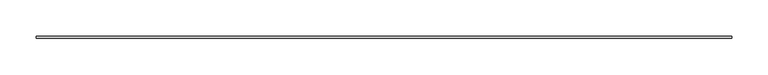
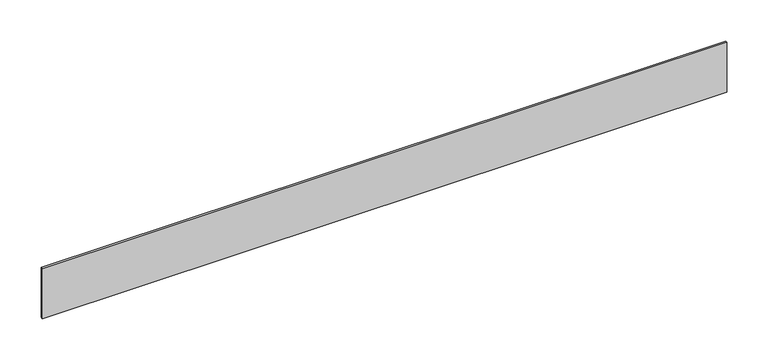
"""IFC4 building model written with IfcOpenShell, lengths in millimetres: proxy geometry, Generic Models 7:Generic Models 1:7:Generic Models 1:7 : Generic Models 7:Generic Models 1:337419:3 : Generic Models 7:Generic Models 1:7:Generic Models 1:7 : Generic Models 7:Generic Models 1:337419:315055."""

from ifc_helpers import new_model, si_unit, frame, origin, place, context, project, spatial, polyline, outline, extrude, source, transform, mapped, element, save


def generic_models_c86f317e(model_context):
    return source(origin(), model_context, "Body", "SweptSolid", [
        extrude(outline(polyline([(570431.3487584, -578997.5163841), (570431.3487584, -579000.6913841), (569470.2262575, -579000.6913841), (569470.2262575, -578997.5163841), (570431.3487584, -578997.5163841)])), frame((0.0, 0.0, 1.8707208), z_axis=(0.0, 0.0, 1.0), x_axis=(1.0, 0.0, 0.0)), (0.0, 0.0, 1.0), 74.3292792),
    ])


if __name__ == "__main__":
    model = new_model("IFC4")
    model_context = context("Model", 3, world=origin())
    ifc_project = project(units=[si_unit("LENGTHUNIT", "METRE", prefix="MILLI")], contexts=[model_context])
    site = spatial("IfcSite", under=ifc_project)
    building = spatial("IfcBuilding", under=site)
    placement = place(None, origin())
    generic_models_shape = generic_models_c86f317e(model_context)
    element("IfcBuildingElementProxy", 1, Name="Generic Models 7:Generic Models 1:7:Generic Models 1:7 : Generic Models 7:Generic Models 1:337419:3 : Generic Models 7:Generic Models 1:7:Generic Models 1:7 : Generic Models 7:Generic Models 1:337419:315055", ObjectType="Generic Models 7:Generic Models 1:7:Generic Models 1:7 : Generic Models 7:Generic Models 1:337419:3 : Generic Models 7:Generic Models 1:7:Generic Models 1:7 : Generic Models 7:Generic Models 1:337419:315055", at=placement, inside=building, context=model_context, shape_type="MappedRepresentation", body=[
        mapped(generic_models_shape, transform((0.0, 0.0, 0.0), x_axis=(1.0, 0.0, 0.0), y_axis=(0.0, 1.0, 0.0), z_axis=(0.0, 0.0, 1.0))),
    ])
    save(model, "model.ifc")

# Revit data of these elements
# Type "Generic Models 7:Generic Models 1:7:Generic Models 1:7 : Generic Models 7:Generic Models 1:337419:3 : Generic Models 7:Generic Models 1:7:Generic Models 1:7 : Generic Models 7:Generic Models 1:337419:315055"
#   NameOverride = "Generic Models 7:Generic Models 1:7:Generic Models 1:7 : Generic Models 7:Generic Models 1:337419:315055"
#   ObjectTypeOverride = "Generic Models 1:7 : Generic Models 7:Generic Models 1:337419"
#   Reference = "Generic Models 1"
#   Tag = "315055"
# Element 1 (IfcBuildingElementProxy, "Generic Models 7:Generic Models 1:7:Generic Models 1:7 : Generic Models 7:Generic Models 1:337419:3 : Generic Models 7:Generic Models 1:7:Generic Models 1:7 : Generic Models 7:Generic Models 1:337419:315055")
#   Materials on its faces: "ALUM. BASE TRIM"
# Materials
#   "ALUM. BASE TRIM": class "Generic", colour RGB 120 120 120, transparency 0, Cost = 0
